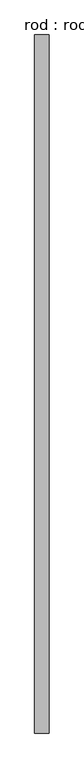
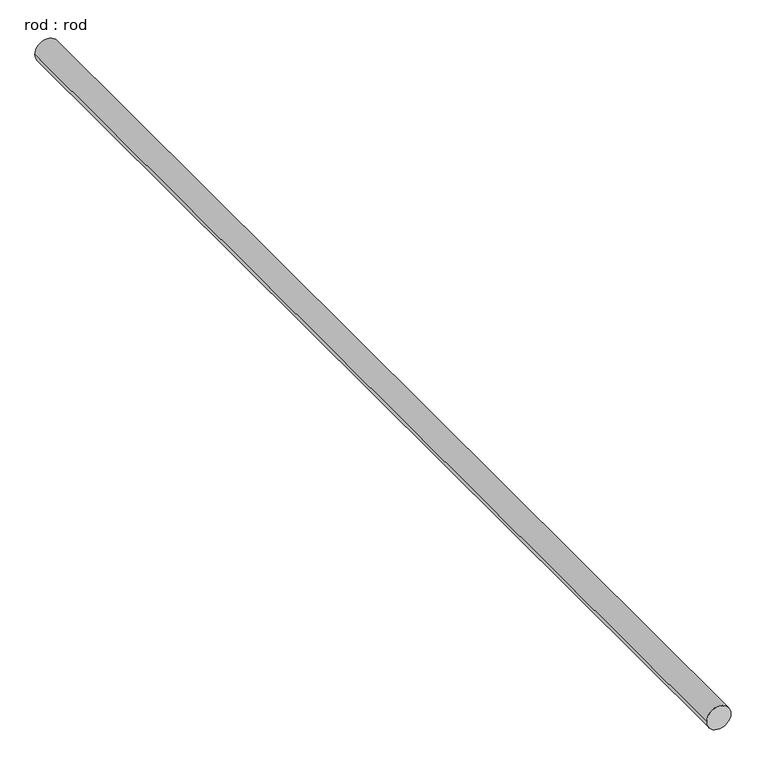
"""IFC4 building model written with IfcOpenShell, lengths in millimetres: proxy geometry, rod : rod."""

from ifc_helpers import new_model, si_unit, point, frame, frame_2d, origin, place, context, project, spatial, circle_curve, trimmed, segment, composite_curve, outline, extrude, source, transform, mapped, element, save


def rod_rod_8ba571e5(model_context):
    return source(origin(), model_context, "Body", "SweptSolid", [
        extrude(outline(composite_curve([segment(trimmed(circle_curve(frame_2d((0.0108462, 0.0)), 200.0), [point((0.0108462, 200.0))], [point((0.0108462, -200.0))], False, "CARTESIAN"), True, "CONTINUOUS"), segment(trimmed(circle_curve(frame_2d((0.0108462, 0.0)), 200.0), [point((0.0108462, -200.0))], [point((0.0108462, 200.0))], False, "CARTESIAN"), True, "CONTINUOUS")], self_intersect=False)), frame((0.0, -5514.407079, 0.0), z_axis=(0.0, 1.0, 0.0), x_axis=(0.0, 0.0, 1.0)), (0.0, 0.0, 1.0), 19214.2713887),
    ])


if __name__ == "__main__":
    model = new_model("IFC4")
    model_context = context("Model", 3, world=origin())
    ifc_project = project(units=[si_unit("LENGTHUNIT", "METRE", prefix="MILLI")], contexts=[model_context])
    site = spatial("IfcSite", under=ifc_project)
    building = spatial("IfcBuilding", under=site)
    placement = place(None, origin())
    rod_rod_shape = rod_rod_8ba571e5(model_context)
    element("IfcBuildingElementProxy", 1, Name="rod : rod", ObjectType="rod : rod", at=placement, inside=building, context=model_context, shape_type="MappedRepresentation", body=[
        mapped(rod_rod_shape, transform((0.0, 0.0, 0.0), x_axis=(1.0, 0.0, 0.0), y_axis=(0.0, 1.0, 0.0), z_axis=(0.0, 0.0, 1.0))),
    ])
    save(model, "model.ifc")

# Revit data of these elements
# Type "rod : rod"
#   Default Elevation = 0
